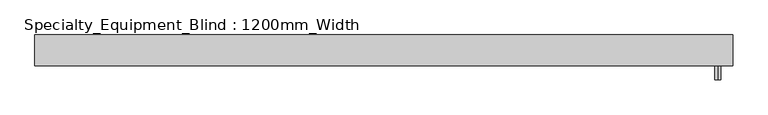
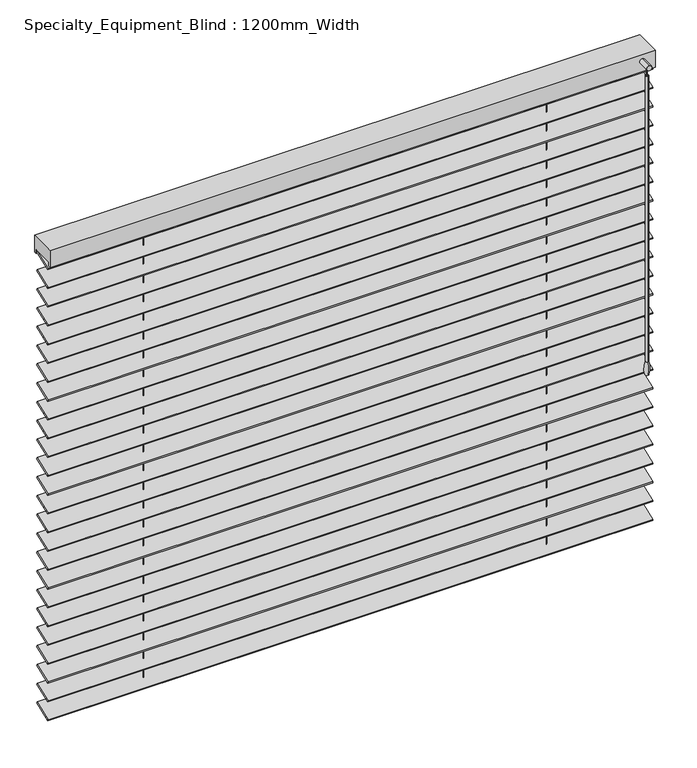
"""IFC4 building model written with IfcOpenShell, lengths in millimetres: proxy geometry, Specialty_Equipment_Blind : 1200mm_Width."""

from ifc_helpers import new_model, si_unit, point, frame, frame_2d, origin, place, context, project, spatial, polyline, circle_curve, ellipse_curve, trimmed, segment, composite_curve, outline, extrude, source, transform, mapped, element, save
from ifc_brep_helpers import plane_surface, cylinder_surface, revolved_surface, advanced_brep


def specialty_equipment_blind_1200mm_width_23c077ca(model_context):
    return source(origin(), model_context, "Body", "SolidModel", [
        extrude(outline(polyline([(0.0, -40.0), (0.0, 0.0), (1180.0, 0.0), (1180.0, -40.0), (0.0, -40.0)])), frame((-439.5079376, 65.0532351, 2040.2125618), z_axis=(0.0, -0.3420201433256684, 0.9396926207859085), x_axis=(1.0, 0.0, 0.0)), (0.0, 0.0, 1.0), 3.0625345),
        extrude(outline(polyline([(0.0, -40.0), (0.0, 0.0), (1180.0, 0.0), (1180.0, -40.0), (0.0, -40.0)])), frame((-439.5079376, 65.0532351, 2001.4625618), z_axis=(0.0, -0.3420201433256684, 0.9396926207859085), x_axis=(1.0, 0.0, 0.0)), (0.0, 0.0, 1.0), 3.0625345),
        extrude(outline(polyline([(0.0, -40.0), (0.0, 0.0), (1180.0, 0.0), (1180.0, -40.0), (0.0, -40.0)])), frame((-439.5079376, 65.0532351, 1962.7125618), z_axis=(0.0, -0.3420201433256684, 0.9396926207859085), x_axis=(1.0, 0.0, 0.0)), (0.0, 0.0, 1.0), 3.0625345),
        extrude(outline(polyline([(0.0, -40.0), (0.0, 0.0), (1180.0, 0.0), (1180.0, -40.0), (0.0, -40.0)])), frame((-439.5079376, 65.0532351, 1923.9625618), z_axis=(0.0, -0.3420201433256684, 0.9396926207859085), x_axis=(1.0, 0.0, 0.0)), (0.0, 0.0, 1.0), 3.0625345),
        extrude(outline(polyline([(0.0, -40.0), (0.0, 0.0), (1180.0, 0.0), (1180.0, -40.0), (0.0, -40.0)])), frame((-439.5079376, 65.0532351, 1885.2125618), z_axis=(0.0, -0.3420201433256684, 0.9396926207859085), x_axis=(1.0, 0.0, 0.0)), (0.0, 0.0, 1.0), 3.0625345),
        extrude(outline(polyline([(0.0, -40.0), (0.0, 0.0), (1180.0, 0.0), (1180.0, -40.0), (0.0, -40.0)])), frame((-439.5079376, 65.0532351, 1846.4625618), z_axis=(0.0, -0.3420201433256684, 0.9396926207859085), x_axis=(1.0, 0.0, 0.0)), (0.0, 0.0, 1.0), 3.0625345),
        extrude(outline(polyline([(0.0, -40.0), (0.0, 0.0), (1180.0, 0.0), (1180.0, -40.0), (0.0, -40.0)])), frame((-439.5079376, 65.0532351, 1807.7125618), z_axis=(0.0, -0.3420201433256684, 0.9396926207859085), x_axis=(1.0, 0.0, 0.0)), (0.0, 0.0, 1.0), 3.0625345),
        extrude(outline(polyline([(0.0, -40.0), (0.0, 0.0), (1180.0, 0.0), (1180.0, -40.0), (0.0, -40.0)])), frame((-439.5079376, 65.0532351, 1768.9625618), z_axis=(0.0, -0.3420201433256684, 0.9396926207859085), x_axis=(1.0, 0.0, 0.0)), (0.0, 0.0, 1.0), 3.0625345),
        extrude(outline(polyline([(0.0, -40.0), (0.0, 0.0), (1180.0, 0.0), (1180.0, -40.0), (0.0, -40.0)])), frame((-439.5079376, 65.0532351, 1730.2125618), z_axis=(0.0, -0.3420201433256684, 0.9396926207859085), x_axis=(1.0, 0.0, 0.0)), (0.0, 0.0, 1.0), 3.0625345),
        extrude(outline(polyline([(0.0, -40.0), (0.0, 0.0), (1180.0, 0.0), (1180.0, -40.0), (0.0, -40.0)])), frame((-439.5079376, 65.0532351, 1691.4625618), z_axis=(0.0, -0.3420201433256684, 0.9396926207859085), x_axis=(1.0, 0.0, 0.0)), (0.0, 0.0, 1.0), 3.0625345),
        extrude(outline(polyline([(0.0, -40.0), (0.0, 0.0), (1180.0, 0.0), (1180.0, -40.0), (0.0, -40.0)])), frame((-439.5079376, 65.0532351, 1652.7125618), z_axis=(0.0, -0.3420201433256684, 0.9396926207859085), x_axis=(1.0, 0.0, 0.0)), (0.0, 0.0, 1.0), 3.0625345),
        extrude(outline(polyline([(0.0, -40.0), (0.0, 0.0), (1180.0, 0.0), (1180.0, -40.0), (0.0, -40.0)])), frame((-439.5079376, 65.0532351, 1613.9625618), z_axis=(0.0, -0.3420201433256684, 0.9396926207859085), x_axis=(1.0, 0.0, 0.0)), (0.0, 0.0, 1.0), 3.0625345),
        extrude(outline(polyline([(0.0, -40.0), (0.0, 0.0), (1180.0, 0.0), (1180.0, -40.0), (0.0, -40.0)])), frame((-439.5079376, 65.0532351, 1575.2125618), z_axis=(0.0, -0.3420201433256684, 0.9396926207859085), x_axis=(1.0, 0.0, 0.0)), (0.0, 0.0, 1.0), 3.0625345),
        extrude(outline(polyline([(0.0, -40.0), (0.0, 0.0), (1180.0, 0.0), (1180.0, -40.0), (0.0, -40.0)])), frame((-439.5079376, 65.0532351, 1536.4625618), z_axis=(0.0, -0.3420201433256684, 0.9396926207859085), x_axis=(1.0, 0.0, 0.0)), (0.0, 0.0, 1.0), 3.0625345),
        extrude(outline(polyline([(0.0, -40.0), (0.0, 0.0), (1180.0, 0.0), (1180.0, -40.0), (0.0, -40.0)])), frame((-439.5079376, 65.0532351, 1497.7125618), z_axis=(0.0, -0.3420201433256684, 0.9396926207859085), x_axis=(1.0, 0.0, 0.0)), (0.0, 0.0, 1.0), 3.0625345),
        extrude(outline(polyline([(0.0, -40.0), (0.0, 0.0), (1180.0, 0.0), (1180.0, -40.0), (0.0, -40.0)])), frame((-439.5079376, 65.0532351, 1458.9625618), z_axis=(0.0, -0.3420201433256684, 0.9396926207859085), x_axis=(1.0, 0.0, 0.0)), (0.0, 0.0, 1.0), 3.0625345),
        extrude(outline(polyline([(0.0, -40.0), (0.0, 0.0), (1180.0, 0.0), (1180.0, -40.0), (0.0, -40.0)])), frame((-439.5079376, 65.0532351, 1420.2125618), z_axis=(0.0, -0.3420201433256684, 0.9396926207859085), x_axis=(1.0, 0.0, 0.0)), (0.0, 0.0, 1.0), 3.0625345),
        extrude(outline(polyline([(0.0, -40.0), (0.0, 0.0), (1180.0, 0.0), (1180.0, -40.0), (0.0, -40.0)])), frame((-439.5079376, 65.0532351, 1381.4625618), z_axis=(0.0, -0.3420201433256684, 0.9396926207859085), x_axis=(1.0, 0.0, 0.0)), (0.0, 0.0, 1.0), 3.0625345),
        extrude(outline(polyline([(0.0, -40.0), (0.0, 0.0), (1180.0, 0.0), (1180.0, -40.0), (0.0, -40.0)])), frame((-439.5079376, 65.0532351, 1342.7125618), z_axis=(0.0, -0.3420201433256684, 0.9396926207859085), x_axis=(1.0, 0.0, 0.0)), (0.0, 0.0, 1.0), 3.0625345),
        extrude(outline(polyline([(0.0, -40.0), (0.0, 0.0), (1180.0, 0.0), (1180.0, -40.0), (0.0, -40.0)])), frame((-439.5079376, 65.0532351, 1303.9625618), z_axis=(0.0, -0.3420201433256684, 0.9396926207859085), x_axis=(1.0, 0.0, 0.0)), (0.0, 0.0, 1.0), 3.0625345),
        extrude(outline(polyline([(0.0, -40.0), (0.0, 0.0), (1180.0, 0.0), (1180.0, -40.0), (0.0, -40.0)])), frame((-439.5079376, 65.0532351, 1265.2125618), z_axis=(0.0, -0.3420201433256684, 0.9396926207859085), x_axis=(1.0, 0.0, 0.0)), (0.0, 0.0, 1.0), 3.0625345),
        extrude(outline(polyline([(0.0, -40.0), (0.0, 0.0), (1180.0, 0.0), (1180.0, -40.0), (0.0, -40.0)])), frame((-439.5079376, 65.0532351, 1226.4625618), z_axis=(0.0, -0.3420201433256684, 0.9396926207859085), x_axis=(1.0, 0.0, 0.0)), (0.0, 0.0, 1.0), 3.0625345),
        extrude(outline(polyline([(0.0, -40.0), (0.0, 0.0), (1180.0, 0.0), (1180.0, -40.0), (0.0, -40.0)])), frame((-439.5079376, 65.0532351, 1187.7125618), z_axis=(0.0, -0.3420201433256684, 0.9396926207859085), x_axis=(1.0, 0.0, 0.0)), (0.0, 0.0, 1.0), 3.0625345),
        extrude(outline(polyline([(0.0, -40.0), (0.0, 0.0), (1180.0, 0.0), (1180.0, -40.0), (0.0, -40.0)])), frame((-439.5079376, 65.0532351, 2078.9625618), z_axis=(0.0, -0.3420201433256684, 0.9396926207859085), x_axis=(1.0, 0.0, 0.0)), (0.0, 0.0, 1.0), 3.0625345),
        extrude(outline(polyline([(0.0, -40.0), (0.0, 0.0), (1180.0, 0.0), (1180.0, -40.0), (0.0, -40.0)])), frame((-439.5079376, 65.0532351, 1148.9625618), z_axis=(0.0, -0.3420201433256684, 0.9396926207859085), x_axis=(1.0, 0.0, 0.0)), (0.0, 0.0, 1.0), 3.0625345),
        extrude(outline(composite_curve([segment(trimmed(circle_curve(frame_2d((-242.8412709, 45.2119342)), 0.5), [point((-243.3412709, 45.2119342))], [point((-242.3412709, 45.2119342))], False, "CARTESIAN"), True, "CONTINUOUS"), segment(trimmed(circle_curve(frame_2d((-242.8412709, 45.2119342)), 0.5), [point((-242.3412709, 45.2119342))], [point((-243.3412709, 45.2119342))], False, "CARTESIAN"), True, "CONTINUOUS")], self_intersect=False)), frame((0.0, 0.0, 1130.0), z_axis=(0.0, 0.0, 1.0), x_axis=(1.0, 0.0, 0.0)), (0.0, 0.0, 1.0), 953.2448883),
        extrude(outline(composite_curve([segment(trimmed(circle_curve(frame_2d((543.8253958, 45.2119342)), 0.5), [point((543.3253958, 45.2119342))], [point((544.3253958, 45.2119342))], False, "CARTESIAN"), True, "CONTINUOUS"), segment(trimmed(circle_curve(frame_2d((543.8253958, 45.2119342)), 0.5), [point((544.3253958, 45.2119342))], [point((543.3253958, 45.2119342))], False, "CARTESIAN"), True, "CONTINUOUS")], self_intersect=False)), frame((0.0, 0.0, 1130.0), z_axis=(0.0, 0.0, 1.0), x_axis=(1.0, 0.0, 0.0)), (0.0, 0.0, 1.0), 953.2448883),
        advanced_brep(
        [(715.4920624, 4.7248495, 2091.3243671), (715.4920624, 2.7248495, 2091.3243671), (715.4920624, 3.7248495, 2091.3243671), (715.4920624, 4.7248495, 2076.3243671), (715.4920624, 2.7248495, 2076.3243671), (715.4920624, 6.7248495, 2076.3243671), (715.4920624, 0.7248495, 2076.3243671), (715.4920624, 6.7248495, 1486.909931), (715.4920624, 0.7248495, 1486.909931), (715.4920624, 7.2513368, 1460.0), (715.4920624, 0.1983622, 1460.0), (715.4920624, 3.7248495, 1460.0)],
        [
            (0, 1, circle_curve(frame((715.4920624, 3.7248495, 2091.3243671), z_axis=(0.0, 0.0, 1.0), x_axis=(0.0, -1.0, 0.0)), 1.0)),
            (1, 2),
            (2, 0),
            (1, 0, circle_curve(frame((715.4920624, 3.7248495, 2091.3243671), z_axis=(0.0, 0.0, 1.0), x_axis=(0.0, -1.0, 0.0)), 1.0)),
            (3, 4, circle_curve(frame((715.4920624, 3.7248495, 2076.3243671), z_axis=(0.0, 0.0, 1.0), x_axis=(0.0, -1.0, 0.0)), 1.0)),
            (4, 1),
            (0, 3),
            (4, 3, circle_curve(frame((715.4920624, 3.7248495, 2076.3243671), z_axis=(0.0, 0.0, 1.0), x_axis=(0.0, -1.0, 0.0)), 1.0)),
            (5, 6, circle_curve(frame((715.4920624, 3.7248495, 2076.3243671), z_axis=(0.0, 0.0, 1.0), x_axis=(0.0, -1.0, 0.0)), 3.0)),
            (6, 4),
            (3, 5),
            (6, 5, circle_curve(frame((715.4920624, 3.7248495, 2076.3243671), z_axis=(0.0, 0.0, 1.0), x_axis=(0.0, -1.0, 0.0)), 3.0)),
            (7, 8, circle_curve(frame((715.4920624, 3.7248495, 1486.909931), z_axis=(0.0, 0.0, 1.0), x_axis=(0.0, -1.0, 0.0)), 3.0)),
            (8, 6),
            (5, 7),
            (8, 7, circle_curve(frame((715.4920624, 3.7248495, 1486.909931), z_axis=(0.0, 0.0, 1.0), x_axis=(0.0, -1.0, 0.0)), 3.0)),
            (9, 10, circle_curve(frame((715.4920624, 3.7248495, 1460.0), z_axis=(0.0, 0.0, 1.0), x_axis=(0.0, -1.0, 0.0)), 3.5264873)),
            (10, 8, circle_curve(frame((715.4920624, 49.2720063, 1472.5), z_axis=(-1.0, 0.0, 0.0), x_axis=(0.0, 1.0, 0.0)), 50.6406214)),
            (7, 9, circle_curve(frame((715.4920624, -41.8223072, 1472.5), z_axis=(-1.0, 0.0, 0.0), x_axis=(0.0, -1.0, 0.0)), 50.6406214)),
            (10, 9, circle_curve(frame((715.4920624, 3.7248495, 1460.0), z_axis=(0.0, 0.0, 1.0), x_axis=(0.0, -1.0, 0.0)), 3.5264873)),
            (11, 10),
            (9, 11),
        ],
        [
            plane_surface(frame((715.4920624, 3.7248495, 2091.3243671), z_axis=(0.0, 0.0, 1.0), x_axis=(0.0, -1.0, 0.0))),
            cylinder_surface(frame((715.4920624, 3.7248495, 1191.3243671), z_axis=(0.0, 0.0, -1.0), x_axis=(0.0, -1.0, 0.0)), 1.0),
            plane_surface(frame((715.4920624, 3.7248495, 2076.3243671), z_axis=(0.0, 0.0, 1.0), x_axis=(0.0, -1.0, 0.0))),
            cylinder_surface(frame((715.4920624, 3.7248495, 1191.3243671), z_axis=(0.0, 0.0, -1.0), x_axis=(0.0, -1.0, 0.0)), 3.0),
            revolved_surface(trimmed(ellipse_curve(frame((715.4920624, 49.2720063, 1472.5), z_axis=(1.0, 0.0, 0.0), x_axis=(0.0, 1.0, 0.0)), 50.6406214, 50.6406214), [point((715.4920624, 0.7248495, 1486.909931))], [point((715.4920624, 0.1983622, 1460.0))], True, "CARTESIAN"), (715.4920624, 3.7248495, 1191.3243671), (0.0, 0.0, -1.0)),
            plane_surface(frame((715.4920624, 3.7248495, 1460.0), z_axis=(0.0, 0.0, -1.0), x_axis=(0.0, -1.0, 0.0))),
        ],
        [
            (0, [[1, 2, 3]]),
            (0, [[4, -3, -2]]),
            (1, [[5, 6, -1, 7]]),
            (1, [[8, -7, -4, -6]]),
            (2, [[9, 10, -5, 11]]),
            (2, [[12, -11, -8, -10]]),
            (3, [[13, 14, -9, 15]]),
            (3, [[16, -15, -12, -14]]),
            (4, [[17, 18, -13, 19]]),
            (4, [[20, -19, -16, -18]]),
            (5, [[21, -17, 22]]),
            (5, [[-22, -20, -21]]),
        ],
    ),
        extrude(outline(composite_curve([segment(trimmed(circle_curve(frame_2d((2095.9171213, 715.4920624)), 5.0), [point((2100.9171213, 715.4920624))], [point((2090.9171213, 715.4920624))], False, "CARTESIAN"), True, "CONTINUOUS"), segment(trimmed(circle_curve(frame_2d((2095.9171213, 715.4920624)), 5.0), [point((2090.9171213, 715.4920624))], [point((2100.9171213, 715.4920624))], False, "CARTESIAN"), True, "CONTINUOUS")], self_intersect=False)), frame((0.0, -4.4512463, 0.0), z_axis=(0.0, 1.0, 0.0), x_axis=(0.0, 0.0, 1.0)), (0.0, 0.0, 1.0), 23.7809602),
        extrude(outline(polyline([(19.329714, 2110.0), (71.0941545, 2110.0), (71.0941545, 2075.0), (66.0941545, 2075.0), (66.0941545, 2083.2448883), (24.329714, 2083.2448883), (24.329714, 2075.0), (19.329714, 2075.0), (19.329714, 2110.0)])), frame((-439.5079376, 0.0, 0.0), z_axis=(1.0, 0.0, 0.0), x_axis=(0.0, 1.0, 0.0)), (0.0, 0.0, 1.0), 1180.0),
    ])


if __name__ == "__main__":
    model = new_model("IFC4")
    model_context = context("Model", 3, world=origin())
    ifc_project = project(units=[si_unit("LENGTHUNIT", "METRE", prefix="MILLI")], contexts=[model_context])
    site = spatial("IfcSite", under=ifc_project)
    building = spatial("IfcBuilding", under=site)
    placement = place(None, origin())
    specialty_equipment_blind_1200mm_width_shape = specialty_equipment_blind_1200mm_width_23c077ca(model_context)
    element("IfcBuildingElementProxy", 1, Name="Specialty_Equipment_Blind : 1200mm_Width", ObjectType="Specialty_Equipment_Blind : 1200mm_Width", at=placement, inside=building, context=model_context, shape_type="MappedRepresentation", body=[
        mapped(specialty_equipment_blind_1200mm_width_shape, transform((0.0, 0.0, 0.0), x_axis=(1.0, 0.0, 0.0), y_axis=(0.0, 1.0, 0.0), z_axis=(0.0, 0.0, 1.0))),
    ])
    save(model, "model.ifc")

# Revit data of these elements
# Type "Specialty_Equipment_Blind : 1200mm_Width"
#   Keynote = "N10/240"
#   Opening Width = 1200 mm
#   End Offset = 10 mm
#   Blind Length = 1180 mm
#   Blind Fixing Height = 2110 mm
#   Blind Depth = 980 mm
#   Blind Angle = 20.00°
#   Blade Depth = 40 mm
#   No of Blades = 25
#   Material Blind = Wood - Birch
# Element 1 (IfcBuildingElementProxy, "Specialty_Equipment_Blind : 1200mm_Width")
#   Materials on its faces: "Wood - Birch"
# Materials
#   "Wood - Birch": class "Wood", colour RGB 224 178 126, transparency 0
